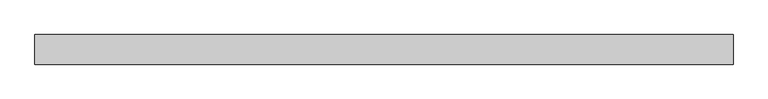
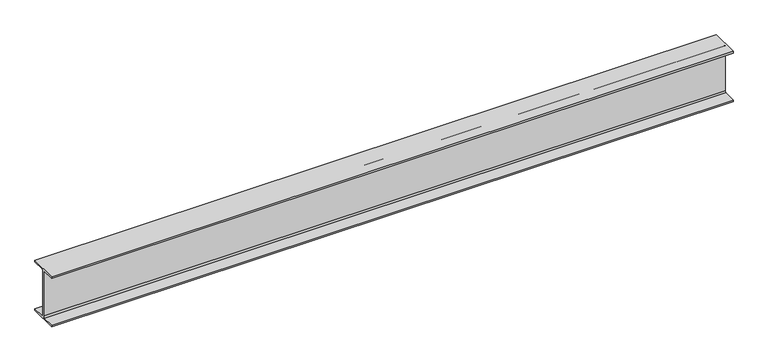
"""IFC4 building model written with IfcOpenShell, lengths in millimetres: beam geometry, Old_Steel Beam_H-KSD3502 : H_SB_ASB_H-250×125x6x9."""

from ifc_helpers import new_model, si_unit, point, frame, frame_2d, origin, place, context, project, spatial, polyline, circle_curve, trimmed, segment, composite_curve, outline, extrude, source, transform, mapped, element, save


def beam_36457d38(model_context):
    return source(origin(), model_context, "Body", "SweptSolid", [
        extrude(outline(composite_curve([segment(polyline([(82.5, -141.5), (82.5, -151.7), (-82.5, -151.7), (-82.5, -141.5), (-11.9, -141.5)]), True, "CONTINUOUS"), segment(trimmed(circle_curve(frame_2d((-11.9, -132.6)), 8.9), [point((-11.9, -141.5))], [point((-3.0, -132.6))], True, "CARTESIAN"), True, "CONTINUOUS"), segment(polyline([(-3.0, -132.6), (-3.0, 132.6)]), True, "CONTINUOUS"), segment(trimmed(circle_curve(frame_2d((-11.9, 132.6)), 8.9), [point((-3.0, 132.6))], [point((-11.9, 141.5))], True, "CARTESIAN"), True, "CONTINUOUS"), segment(polyline([(-11.9, 141.5), (-82.5, 141.5), (-82.5, 151.7), (82.5, 151.7), (82.5, 141.5), (11.9, 141.5)]), True, "CONTINUOUS"), segment(trimmed(circle_curve(frame_2d((11.9, 132.6)), 8.9), [point((11.9, 141.5))], [point((3.0, 132.6))], True, "CARTESIAN"), True, "CONTINUOUS"), segment(polyline([(3.0, 132.6), (3.0, -132.6)]), True, "CONTINUOUS"), segment(trimmed(circle_curve(frame_2d((11.9, -132.6)), 8.9), [point((3.0, -132.6))], [point((11.9, -141.5))], True, "CARTESIAN"), True, "CONTINUOUS"), segment(polyline([(11.9, -141.5), (82.5, -141.5)]), True, "CONTINUOUS")], self_intersect=False)), frame((-1904.8, 0.0, 0.0), z_axis=(1.0, 0.0, 0.0), x_axis=(0.0, 1.0, 0.0)), (0.0, 0.0, 1.0), 3892.0999994),
    ])


if __name__ == "__main__":
    model = new_model("IFC4")
    model_context = context("Model", 3, world=origin())
    ifc_project = project(units=[si_unit("LENGTHUNIT", "METRE", prefix="MILLI")], contexts=[model_context])
    site = spatial("IfcSite", under=ifc_project)
    building = spatial("IfcBuilding", under=site)
    placement = place(None, origin())
    beam_shape = beam_36457d38(model_context)
    element("IfcBeam", 1, ObjectType="Old_Steel Beam_H-KSD3502 : H_SB_ASB_H-250×125x6x9", at=placement, inside=building, context=model_context, shape_type="MappedRepresentation", body=[
        mapped(beam_shape, transform((0.0, 0.0, 0.0), x_axis=(1.0, 0.0, 0.0), y_axis=(0.0, 1.0, 0.0), z_axis=(0.0, 0.0, 1.0))),
    ])
    save(model, "model.ifc")

# Revit data of these elements
# Type "Old_Steel Beam_H-KSD3502 : H_SB_ASB_H-250×125x6x9"
#   Width = 12.5 cm
#   Web Thickness = 0.6 cm
#   Web Fillet = 1.2 cm
#   Warping Constant = 42539.8 cm⁶
#   Torsional Moment of Inertia = 7.8102 cm⁴
#   Torsional Modulus = 1.0 cm³
#   Section Area = 37.66 cm²
#   Plastic Modulus weak axis = 73.1 cm³
#   Plastic Modulus strong axis = 366.0 cm³
#   Perimeter = 0.97 m²/m
#   Nominal Weight = 29.60 kgf/m
#   Moment of Inertia weak axis = 294.00 cm⁴
#   Moment of Inertia strong axis = 4050.00 cm⁴
#   Height = 25.0 cm
#   Flange Thickness = 0.9 cm
#   Elastic Modulus weak axis = 47.0 cm³
#   Elastic Modulus strong axis = 324.0 cm³
#   Centroid Vertical = 12.5 cm
#   Centroid Horizontal = 6.25 cm
#   Length [instance default] = 1.5240 m
#   Structural Material [instance default] = Steel, 45-345
#   Assembly Code = ""
# Element 1 (IfcBeam, "Old_Steel Beam_H-KSD3502 : H_SB_ASB_H-250×125x6x9")
#   Structural Material = none
# Materials
#   "Steel, 45-345": class "Metal", colour RGB 189 187 185, transparency 0, Description = "Steel 345 MPa", Cost = 0
